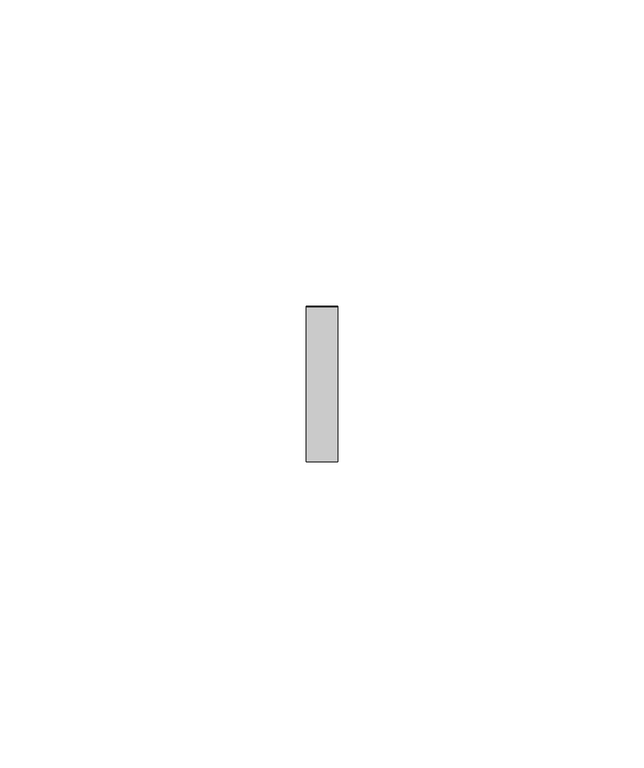
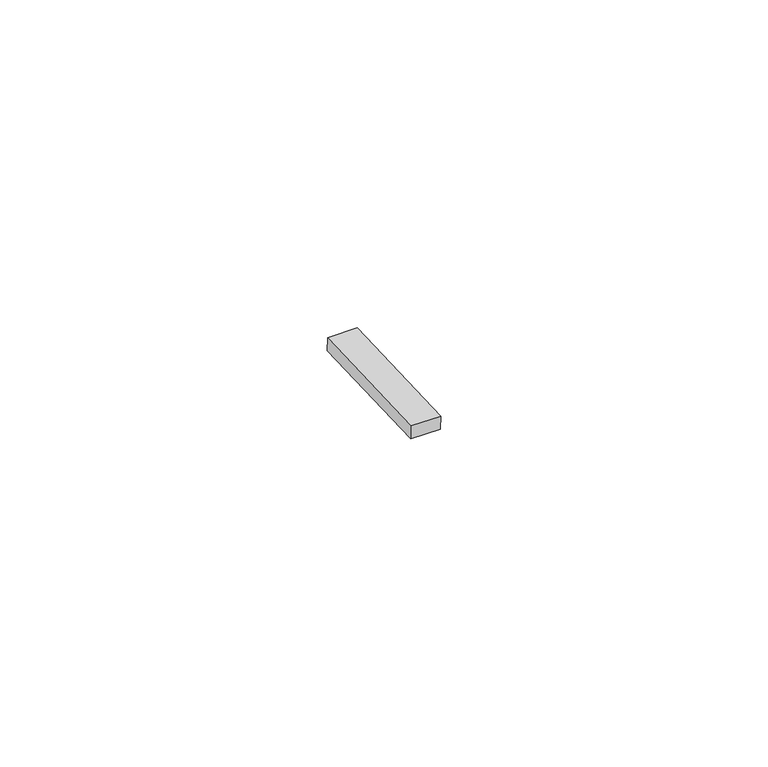
"""IFC4 building model written with IfcOpenShell, lengths in millimetres: proxy geometry, Inner panel:Inner panel:1:Inner panel:1 : Inner panel:Inner panel:300324:2:Inner panel:1:Inner panel:1 : Inner panel:Inner panel:300324:2 : Inner panel:Inner panel:1:Inner panel:1 : Inner panel:Inner panel:300324:300043:106 : Inner panel:Inner panel:1:Inner panel:1 : Inner panel:Inner panel:300324:2:Inner panel:1:Inner panel:1 : Inner panel:Inner panel:300324:2 : Inner panel:Inner panel:1:Inner panel:1 : Inner panel:Inner panel:300324:300043:308120."""

import ifcopenshell
import ifcopenshell.guid

model = None  # the IFC model being written
_history = None  # IfcOwnerHistory: only IFC2X3 demands one
_inside = {}  # id of a spatial element -> (the spatial element, [elements in it])
_under = {}  # id of a project, library or spatial element -> (it, [spatial elements below it])
_declared = {}  # id of a project -> (the project, [libraries it declares])
_typed = {}  # id of a type object -> (the type object, [elements of that type])
_made_of = {}  # id of a material, layer set ... -> (it, [elements and type objects made of it])


def new_model(schema):
    """Start an empty IFC model of exactly this schema.

    Asked for "IFC4X3", IfcOpenShell would pick the latest addendum, in which some entities
    have other attributes; the version numbers below select the first issue.
    IFC2X3 requires an IfcOwnerHistory on every rooted entity: one is made here for all.
    """
    global model, _history
    if schema == "IFC4X3":
        model = ifcopenshell.file(schema_version=(4, 3, 0, 0))
    else:
        model = ifcopenshell.file(schema=schema)
    _inside.clear()
    _under.clear()
    _declared.clear()
    _typed.clear()
    _made_of.clear()
    _history = None
    if model.schema == "IFC2X3":
        org = make("IfcOrganization", Name="unknown")
        user = make(
            "IfcPersonAndOrganization",
            ThePerson=make("IfcPerson", FamilyName="unknown"),
            TheOrganization=org,
        )
        app = make(
            "IfcApplication",
            ApplicationDeveloper=org,
            Version="unknown",
            ApplicationFullName="unknown",
            ApplicationIdentifier="unknown",
        )
        _history = make(
            "IfcOwnerHistory",
            OwningUser=user,
            OwningApplication=app,
            ChangeAction="ADDED",
            CreationDate=0,
        )
    return model


def make(cls, **values):
    """One entity of the class cls with the attributes given. An attribute that is None is left unset."""
    return model.create_entity(
        cls, **{name: value for name, value in values.items() if value is not None}
    )


def rooted(cls, **values):
    """An entity with a GlobalId (a new one), such as an element, a storey or a relation."""
    return make(cls, GlobalId=ifcopenshell.guid.new(), OwnerHistory=_history, **values)


def si_unit(unit_type, name, prefix=None):
    """IfcSIUnit, for example si_unit("LENGTHUNIT", "METRE", prefix="MILLI")."""
    return make("IfcSIUnit", UnitType=unit_type, Prefix=prefix, Name=name)


def assignment(units):
    """IfcUnitAssignment: the units of a project."""
    return None if units is None else make("IfcUnitAssignment", Units=units)


def point(xyz):
    """IfcCartesianPoint."""
    return None if xyz is None else make("IfcCartesianPoint", Coordinates=xyz)


def direction(xyz):
    """IfcDirection."""
    return None if xyz is None else make("IfcDirection", DirectionRatios=xyz)


def frame(location, z_axis=None, x_axis=None):
    """IfcAxis2Placement3D, a coordinate frame: its origin and axes. An axis left out is left unset."""
    return make(
        "IfcAxis2Placement3D",
        Location=point(location),
        Axis=direction(z_axis),
        RefDirection=direction(x_axis),
    )


def origin():
    """The frame at (0, 0, 0) with its axes left unset."""
    return frame((0.0, 0.0, 0.0))


def place(relative_to, where):
    """IfcLocalPlacement: puts the frame where relative to a parent placement (None: the world)."""
    return make(
        "IfcLocalPlacement", PlacementRelTo=relative_to, RelativePlacement=where
    )


def context(
    kind, dimensions, precision=None, world=None, true_north=None, identifier=None
):
    """IfcGeometricRepresentationContext, for example the 3D "Model" context."""
    return make(
        "IfcGeometricRepresentationContext",
        ContextIdentifier=identifier,
        ContextType=kind,
        CoordinateSpaceDimension=dimensions,
        Precision=precision,
        WorldCoordinateSystem=world,
        TrueNorth=true_north,
    )


def project(units=None, contexts=None):
    """IfcProject with its units and contexts."""
    return rooted(
        "IfcProject",
        Name="project",
        RepresentationContexts=contexts,
        UnitsInContext=assignment(units),
    )


def spatial(cls, under=None, at=None, **own):
    """A site, building, storey or space (cls), placed at a placement, below another one or the project."""
    s = rooted(cls, ObjectPlacement=at, **own)
    if under is not None:
        _under.setdefault(under.id(), (under, []))[1].append(s)
    return s


def polyline(points):
    """IfcPolyline through the points."""
    return make("IfcPolyline", Points=[point(p) for p in points])


def outline(outer, holes=None, kind="AREA"):
    """IfcArbitraryClosedProfileDef: a profile drawn as a closed curve; with holes, ...WithVoids."""
    if holes is None:
        return make("IfcArbitraryClosedProfileDef", ProfileType=kind, OuterCurve=outer)
    return make(
        "IfcArbitraryProfileDefWithVoids",
        ProfileType=kind,
        OuterCurve=outer,
        InnerCurves=holes,
    )


def extrude(swept, where, along, depth):
    """IfcExtrudedAreaSolid: the profile swept, set in the frame where, extruded along a direction by depth."""
    return make(
        "IfcExtrudedAreaSolid",
        SweptArea=swept,
        Position=where,
        ExtrudedDirection=direction(along),
        Depth=depth,
    )


def shape(context_of_items, identifier, shape_type, items):
    """IfcShapeRepresentation: the items that make up one representation, for example the "Body"."""
    return make(
        "IfcShapeRepresentation",
        ContextOfItems=context_of_items,
        RepresentationIdentifier=identifier,
        RepresentationType=shape_type,
        Items=items,
    )


def source(mapping_origin, context_of_items, identifier, shape_type, items):
    """IfcRepresentationMap: a shape defined once, which mapped items show again and again."""
    return make(
        "IfcRepresentationMap",
        MappingOrigin=mapping_origin,
        MappedRepresentation=shape(context_of_items, identifier, shape_type, items),
    )


def transform(
    local_origin,
    x_axis=None,
    y_axis=None,
    z_axis=None,
    scale=None,
    scale2=None,
    scale3=None,
    uniform=True,
):
    """IfcCartesianTransformationOperator3D, or its non-uniform kind. x_axis, y_axis, z_axis: its Axis1, 2, 3."""
    if uniform:
        return make(
            "IfcCartesianTransformationOperator3D",
            Axis1=direction(x_axis),
            Axis2=direction(y_axis),
            LocalOrigin=point(local_origin),
            Scale=scale,
            Axis3=direction(z_axis),
        )
    return make(
        "IfcCartesianTransformationOperator3DnonUniform",
        Axis1=direction(x_axis),
        Axis2=direction(y_axis),
        LocalOrigin=point(local_origin),
        Scale=scale,
        Axis3=direction(z_axis),
        Scale2=scale2,
        Scale3=scale3,
    )


def mapped(mapping_source, mapping_target):
    """IfcMappedItem: shows the shape of a source again, moved by a transform."""
    return make(
        "IfcMappedItem", MappingSource=mapping_source, MappingTarget=mapping_target
    )


def made_of(thing, what):
    """Note that an element or type object is made of a material, layer set ...; save() writes the relation."""
    if what is not None:
        _made_of.setdefault(what.id(), (what, []))[1].append(thing)
    return thing


def element(
    cls,
    number,
    at=None,
    inside=None,
    cuts=None,
    type_object=None,
    material=None,
    context=None,
    identifier="Body",
    shape_type=None,
    held_by="IfcProductDefinitionShape",
    body=None,
    shapes=None,
    **own,
):
    """One element of the class cls, such as IfcWall. Its Tag is "e" and its number.

    at: its placement. inside: the storey or other place that contains it. cuts: it is an
    opening in that element (IfcRelVoidsElement). A single representation is given by context,
    identifier, shape_type and body (its items); several are given by shapes. held_by: the class
    of the entity that holds the representations. save() writes the other relations.
    """
    e = rooted(cls, Tag="e%d" % number, ObjectPlacement=at, **own)
    if body is not None:
        shapes = [shape(context, identifier, shape_type, body)]
    if shapes is not None:
        e.Representation = make(held_by, Representations=shapes)
    if inside is not None:
        _inside.setdefault(inside.id(), (inside, []))[1].append(e)
    if cuts is not None:
        rooted(
            "IfcRelVoidsElement", RelatingBuildingElement=cuts, RelatedOpeningElement=e
        )
    if type_object is not None:
        _typed.setdefault(type_object.id(), (type_object, []))[1].append(e)
    return made_of(e, material)


def aggregate(whole, parts):
    """IfcRelAggregates: a whole, such as a stair, and the parts it consists of."""
    return rooted("IfcRelAggregates", RelatingObject=whole, RelatedObjects=parts)


def save(model, path):
    """Write the relations noted so far, then the file.

    IfcRelAggregates (storeys below a building ...), IfcRelContainedInSpatialStructure (elements
    in a storey), IfcRelDefinesByType, IfcRelAssociatesMaterial and IfcRelDeclares: one each for
    every whole, place, type object, material and project.
    """
    for whole, parts in _under.values():
        aggregate(whole, parts)
    for where, things in _inside.values():
        rooted(
            "IfcRelContainedInSpatialStructure",
            RelatedElements=things,
            RelatingStructure=where,
        )
    for kind, things in _typed.values():
        rooted("IfcRelDefinesByType", RelatedObjects=things, RelatingType=kind)
    for what, things in _made_of.values():
        rooted("IfcRelAssociatesMaterial", RelatedObjects=things, RelatingMaterial=what)
    for by, libraries in _declared.values():
        rooted("IfcRelDeclares", RelatingContext=by, RelatedDefinitions=libraries)
    model.write(path)


def generic_models_21e38ae0(model_context):
    return source(origin(), model_context, "Body", "SweptSolid", [
        extrude(outline(polyline([(0.0, -25.4), (0.0, 0.0), (5.2138089, 0.0), (5.2138089, -25.4), (0.0, -25.4)])), frame((593530.195117, -578253.2828061, 3981.0403755), z_axis=(0.0, -0.041630544712223896, 0.9991330730923502), x_axis=(-1.0, 0.0, 0.0)), (0.0, 0.0, 1.0), 2.4763745),
    ])


if __name__ == "__main__":
    model = new_model("IFC4")
    model_context = context("Model", 3, world=origin())
    ifc_project = project(units=[si_unit("LENGTHUNIT", "METRE", prefix="MILLI")], contexts=[model_context])
    site = spatial("IfcSite", under=ifc_project)
    building = spatial("IfcBuilding", under=site)
    placement = place(None, origin())
    generic_models_shape = generic_models_21e38ae0(model_context)
    element("IfcBuildingElementProxy", 1, Name="Inner panel:Inner panel:1:Inner panel:1 : Inner panel:Inner panel:300324:2:Inner panel:1:Inner panel:1 : Inner panel:Inner panel:300324:2 : Inner panel:Inner panel:1:Inner panel:1 : Inner panel:Inner panel:300324:300043:106 : Inner panel:Inner panel:1:Inner panel:1 : Inner panel:Inner panel:300324:2:Inner panel:1:Inner panel:1 : Inner panel:Inner panel:300324:2 : Inner panel:Inner panel:1:Inner panel:1 : Inner panel:Inner panel:300324:300043:308120", ObjectType="Inner panel:Inner panel:1:Inner panel:1 : Inner panel:Inner panel:300324:2:Inner panel:1:Inner panel:1 : Inner panel:Inner panel:300324:2 : Inner panel:Inner panel:1:Inner panel:1 : Inner panel:Inner panel:300324:300043:106 : Inner panel:Inner panel:1:Inner panel:1 : Inner panel:Inner panel:300324:2:Inner panel:1:Inner panel:1 : Inner panel:Inner panel:300324:2 : Inner panel:Inner panel:1:Inner panel:1 : Inner panel:Inner panel:300324:300043:308120", at=placement, inside=building, context=model_context, shape_type="MappedRepresentation", body=[
        mapped(generic_models_shape, transform((0.0, 0.0, 0.0), x_axis=(1.0, 0.0, 0.0), y_axis=(0.0, 1.0, 0.0), z_axis=(0.0, 0.0, 1.0))),
    ])
    save(model, "model.ifc")

# Revit data of these elements
# Type "Inner panel:Inner panel:1:Inner panel:1 : Inner panel:Inner panel:300324:2:Inner panel:1:Inner panel:1 : Inner panel:Inner panel:300324:2 : Inner panel:Inner panel:1:Inner panel:1 : Inner panel:Inner panel:300324:300043:106 : Inner panel:Inner panel:1:Inner panel:1 : Inner panel:Inner panel:300324:2:Inner panel:1:Inner panel:1 : Inner panel:Inner panel:300324:2 : Inner panel:Inner panel:1:Inner panel:1 : Inner panel:Inner panel:300324:300043:308120"
#   NameOverride = "Inner panel:Inner panel:1:Inner panel:1 : Inner panel:Inner panel:300324:2:Inner panel:1:Inner panel:1 : Inner panel:Inner panel:300324:2 : Inner panel:Inner panel:1:Inner panel:1 : Inner panel:Inner panel:300324:300043:308120"
#   ObjectTypeOverride = "Inner panel:1:Inner panel:1 : Inner panel:Inner panel:300324:2 : Inner panel:Inner panel:1:Inner panel:1 : Inner panel:Inner panel:300324:300043"
#   Reference = "Inner panel"
#   Tag = "308120"
# Element 1 (IfcBuildingElementProxy, "Inner panel:Inner panel:1:Inner panel:1 : Inner panel:Inner panel:300324:2:Inner panel:1:Inner panel:1 : Inner panel:Inner panel:300324:2 : Inner panel:Inner panel:1:Inner panel:1 : Inner panel:Inner panel:300324:300043:106 : Inner panel:Inner panel:1:Inner panel:1 : Inner panel:Inner panel:300324:2:Inner panel:1:Inner panel:1 : Inner panel:Inner panel:300324:2 : Inner panel:Inner panel:1:Inner panel:1 : Inner panel:Inner panel:300324:300043:308120")
#   Materials on its faces: "AT CLIP - 1\" WIDE NON ABSORBENT, WEATHER-RESISTANT NEOPRENE/EPDM/SBR FOAM"
# Materials
#   "AT CLIP - 1\" WIDE NON ABSORBENT, WEATHER-RESISTANT NEOPRENE/EPDM/SBR FOAM": class "Generic", colour RGB 85 85 85, transparency 0, Cost = 0
